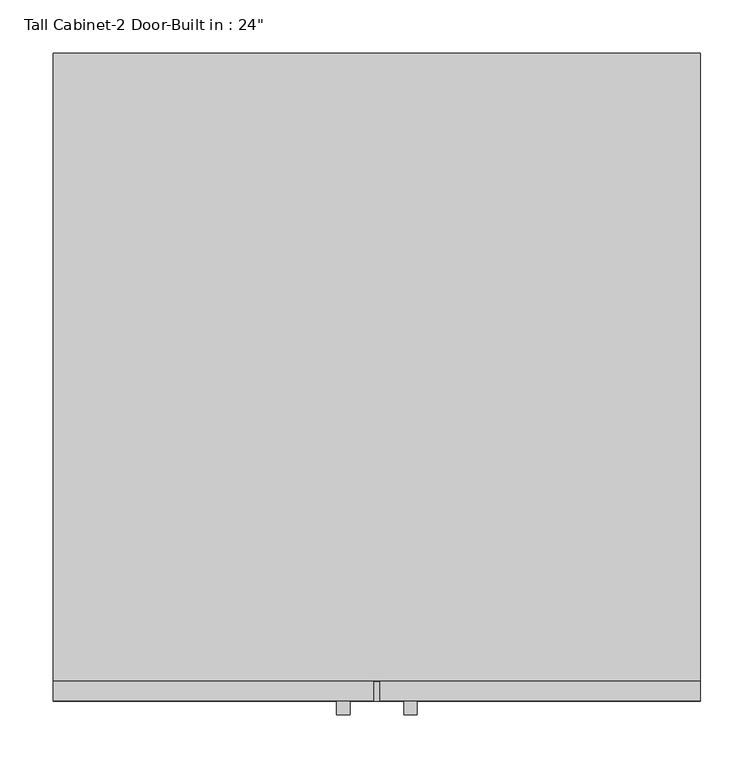
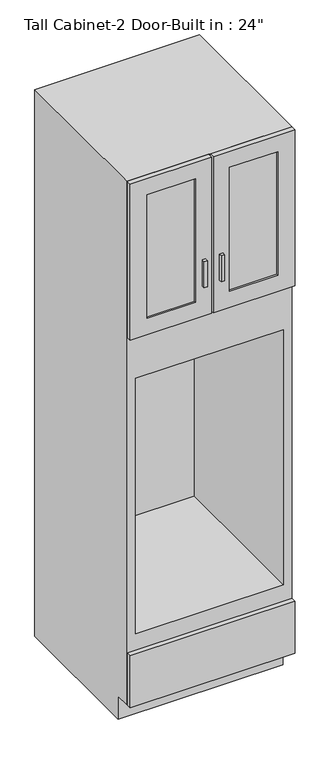
"""IFC4 building model written with IfcOpenShell, lengths in millimetres: furniture geometry."""

import ifcopenshell
import ifcopenshell.guid

model = None  # the IFC model being written
_history = None  # IfcOwnerHistory: only IFC2X3 demands one
_inside = {}  # id of a spatial element -> (the spatial element, [elements in it])
_under = {}  # id of a project, library or spatial element -> (it, [spatial elements below it])
_declared = {}  # id of a project -> (the project, [libraries it declares])
_typed = {}  # id of a type object -> (the type object, [elements of that type])
_made_of = {}  # id of a material, layer set ... -> (it, [elements and type objects made of it])


def new_model(schema):
    """Start an empty IFC model of exactly this schema.

    Asked for "IFC4X3", IfcOpenShell would pick the latest addendum, in which some entities
    have other attributes; the version numbers below select the first issue.
    IFC2X3 requires an IfcOwnerHistory on every rooted entity: one is made here for all.
    """
    global model, _history
    if schema == "IFC4X3":
        model = ifcopenshell.file(schema_version=(4, 3, 0, 0))
    else:
        model = ifcopenshell.file(schema=schema)
    _inside.clear()
    _under.clear()
    _declared.clear()
    _typed.clear()
    _made_of.clear()
    _history = None
    if model.schema == "IFC2X3":
        org = make("IfcOrganization", Name="unknown")
        user = make(
            "IfcPersonAndOrganization",
            ThePerson=make("IfcPerson", FamilyName="unknown"),
            TheOrganization=org,
        )
        app = make(
            "IfcApplication",
            ApplicationDeveloper=org,
            Version="unknown",
            ApplicationFullName="unknown",
            ApplicationIdentifier="unknown",
        )
        _history = make(
            "IfcOwnerHistory",
            OwningUser=user,
            OwningApplication=app,
            ChangeAction="ADDED",
            CreationDate=0,
        )
    return model


def make(cls, **values):
    """One entity of the class cls with the attributes given. An attribute that is None is left unset."""
    return model.create_entity(
        cls, **{name: value for name, value in values.items() if value is not None}
    )


def rooted(cls, **values):
    """An entity with a GlobalId (a new one), such as an element, a storey or a relation."""
    return make(cls, GlobalId=ifcopenshell.guid.new(), OwnerHistory=_history, **values)


def si_unit(unit_type, name, prefix=None):
    """IfcSIUnit, for example si_unit("LENGTHUNIT", "METRE", prefix="MILLI")."""
    return make("IfcSIUnit", UnitType=unit_type, Prefix=prefix, Name=name)


def assignment(units):
    """IfcUnitAssignment: the units of a project."""
    return None if units is None else make("IfcUnitAssignment", Units=units)


def point(xyz):
    """IfcCartesianPoint."""
    return None if xyz is None else make("IfcCartesianPoint", Coordinates=xyz)


def direction(xyz):
    """IfcDirection."""
    return None if xyz is None else make("IfcDirection", DirectionRatios=xyz)


def frame(location, z_axis=None, x_axis=None):
    """IfcAxis2Placement3D, a coordinate frame: its origin and axes. An axis left out is left unset."""
    return make(
        "IfcAxis2Placement3D",
        Location=point(location),
        Axis=direction(z_axis),
        RefDirection=direction(x_axis),
    )


def origin():
    """The frame at (0, 0, 0) with its axes left unset."""
    return frame((0.0, 0.0, 0.0))


def place(relative_to, where):
    """IfcLocalPlacement: puts the frame where relative to a parent placement (None: the world)."""
    return make(
        "IfcLocalPlacement", PlacementRelTo=relative_to, RelativePlacement=where
    )


def context(
    kind, dimensions, precision=None, world=None, true_north=None, identifier=None
):
    """IfcGeometricRepresentationContext, for example the 3D "Model" context."""
    return make(
        "IfcGeometricRepresentationContext",
        ContextIdentifier=identifier,
        ContextType=kind,
        CoordinateSpaceDimension=dimensions,
        Precision=precision,
        WorldCoordinateSystem=world,
        TrueNorth=true_north,
    )


def project(units=None, contexts=None):
    """IfcProject with its units and contexts."""
    return rooted(
        "IfcProject",
        Name="project",
        RepresentationContexts=contexts,
        UnitsInContext=assignment(units),
    )


def spatial(cls, under=None, at=None, **own):
    """A site, building, storey or space (cls), placed at a placement, below another one or the project."""
    s = rooted(cls, ObjectPlacement=at, **own)
    if under is not None:
        _under.setdefault(under.id(), (under, []))[1].append(s)
    return s


def polyline(points):
    """IfcPolyline through the points."""
    return make("IfcPolyline", Points=[point(p) for p in points])


def outline(outer, holes=None, kind="AREA"):
    """IfcArbitraryClosedProfileDef: a profile drawn as a closed curve; with holes, ...WithVoids."""
    if holes is None:
        return make("IfcArbitraryClosedProfileDef", ProfileType=kind, OuterCurve=outer)
    return make(
        "IfcArbitraryProfileDefWithVoids",
        ProfileType=kind,
        OuterCurve=outer,
        InnerCurves=holes,
    )


def extrude(swept, where, along, depth):
    """IfcExtrudedAreaSolid: the profile swept, set in the frame where, extruded along a direction by depth."""
    return make(
        "IfcExtrudedAreaSolid",
        SweptArea=swept,
        Position=where,
        ExtrudedDirection=direction(along),
        Depth=depth,
    )


def faces_of(points, faces, orient=None, outer=None):
    """IfcFace entities. A face is a list of loops; a loop is a list of indices into points, from 0.

    orient and outer hold one flag for each loop. By default every Orientation is true, the
    first loop of a face is its IfcFaceOuterBound and the others are IfcFaceBound.
    """
    made = []
    for i, loops in enumerate(faces):
        bounds = []
        for j, loop in enumerate(loops):
            is_outer = j == 0 if outer is None else outer[i][j]
            bounds.append(
                make(
                    "IfcFaceOuterBound" if is_outer else "IfcFaceBound",
                    Bound=make("IfcPolyLoop", Polygon=[points[k] for k in loop]),
                    Orientation=True if orient is None else orient[i][j],
                )
            )
        made.append(make("IfcFace", Bounds=bounds))
    return made


def faceted_brep(points, faces, orient=None, outer=None, voids=None):
    """IfcFacetedBrep: a solid bounded by flat faces; with voids (closed shells), ...WithVoids."""
    shared = [point(p) for p in points]
    hull = make("IfcClosedShell", CfsFaces=faces_of(shared, faces, orient, outer))
    if voids is None:
        return make("IfcFacetedBrep", Outer=hull)
    return make(
        "IfcFacetedBrepWithVoids",
        Outer=hull,
        Voids=[
            make(cls, CfsFaces=faces_of(shared, fs, o, b)) for cls, fs, o, b in voids
        ],
    )


def shape(context_of_items, identifier, shape_type, items):
    """IfcShapeRepresentation: the items that make up one representation, for example the "Body"."""
    return make(
        "IfcShapeRepresentation",
        ContextOfItems=context_of_items,
        RepresentationIdentifier=identifier,
        RepresentationType=shape_type,
        Items=items,
    )


def source(mapping_origin, context_of_items, identifier, shape_type, items):
    """IfcRepresentationMap: a shape defined once, which mapped items show again and again."""
    return make(
        "IfcRepresentationMap",
        MappingOrigin=mapping_origin,
        MappedRepresentation=shape(context_of_items, identifier, shape_type, items),
    )


def transform(
    local_origin,
    x_axis=None,
    y_axis=None,
    z_axis=None,
    scale=None,
    scale2=None,
    scale3=None,
    uniform=True,
):
    """IfcCartesianTransformationOperator3D, or its non-uniform kind. x_axis, y_axis, z_axis: its Axis1, 2, 3."""
    if uniform:
        return make(
            "IfcCartesianTransformationOperator3D",
            Axis1=direction(x_axis),
            Axis2=direction(y_axis),
            LocalOrigin=point(local_origin),
            Scale=scale,
            Axis3=direction(z_axis),
        )
    return make(
        "IfcCartesianTransformationOperator3DnonUniform",
        Axis1=direction(x_axis),
        Axis2=direction(y_axis),
        LocalOrigin=point(local_origin),
        Scale=scale,
        Axis3=direction(z_axis),
        Scale2=scale2,
        Scale3=scale3,
    )


def mapped(mapping_source, mapping_target):
    """IfcMappedItem: shows the shape of a source again, moved by a transform."""
    return make(
        "IfcMappedItem", MappingSource=mapping_source, MappingTarget=mapping_target
    )


def made_of(thing, what):
    """Note that an element or type object is made of a material, layer set ...; save() writes the relation."""
    if what is not None:
        _made_of.setdefault(what.id(), (what, []))[1].append(thing)
    return thing


def element(
    cls,
    number,
    at=None,
    inside=None,
    cuts=None,
    type_object=None,
    material=None,
    context=None,
    identifier="Body",
    shape_type=None,
    held_by="IfcProductDefinitionShape",
    body=None,
    shapes=None,
    **own,
):
    """One element of the class cls, such as IfcWall. Its Tag is "e" and its number.

    at: its placement. inside: the storey or other place that contains it. cuts: it is an
    opening in that element (IfcRelVoidsElement). A single representation is given by context,
    identifier, shape_type and body (its items); several are given by shapes. held_by: the class
    of the entity that holds the representations. save() writes the other relations.
    """
    e = rooted(cls, Tag="e%d" % number, ObjectPlacement=at, **own)
    if body is not None:
        shapes = [shape(context, identifier, shape_type, body)]
    if shapes is not None:
        e.Representation = make(held_by, Representations=shapes)
    if inside is not None:
        _inside.setdefault(inside.id(), (inside, []))[1].append(e)
    if cuts is not None:
        rooted(
            "IfcRelVoidsElement", RelatingBuildingElement=cuts, RelatedOpeningElement=e
        )
    if type_object is not None:
        _typed.setdefault(type_object.id(), (type_object, []))[1].append(e)
    return made_of(e, material)


def aggregate(whole, parts):
    """IfcRelAggregates: a whole, such as a stair, and the parts it consists of."""
    return rooted("IfcRelAggregates", RelatingObject=whole, RelatedObjects=parts)


def save(model, path):
    """Write the relations noted so far, then the file.

    IfcRelAggregates (storeys below a building ...), IfcRelContainedInSpatialStructure (elements
    in a storey), IfcRelDefinesByType, IfcRelAssociatesMaterial and IfcRelDeclares: one each for
    every whole, place, type object, material and project.
    """
    for whole, parts in _under.values():
        aggregate(whole, parts)
    for where, things in _inside.values():
        rooted(
            "IfcRelContainedInSpatialStructure",
            RelatedElements=things,
            RelatingStructure=where,
        )
    for kind, things in _typed.values():
        rooted("IfcRelDefinesByType", RelatedObjects=things, RelatingType=kind)
    for what, things in _made_of.values():
        rooted("IfcRelAssociatesMaterial", RelatedObjects=things, RelatingMaterial=what)
    for by, libraries in _declared.values():
        rooted("IfcRelDeclares", RelatingContext=by, RelatedDefinitions=libraries)
    model.write(path)


def furniture_1eba2136(model_context):
    return source(origin(), model_context, "Body", "SolidModel", [
        faceted_brep([(323.5377049, -590.55, 90.4875), (323.5377049, -590.55, 2135.1875), (-286.0622951, -590.55, 2135.1875), (-286.0622951, -590.55, 90.4875), (-267.0122951, -590.55, 2116.1375), (304.4877049, -590.55, 2116.1375), (304.4877049, -590.55, 1525.5875), (-267.0122951, -590.55, 1525.5875), (291.7877049, -590.55, 357.1875), (-254.3122951, -590.55, 357.1875), (-254.3122951, -590.55, 1354.1375), (291.7877049, -590.55, 1354.1375), (-286.0622951, 0.0, 2135.1875), (323.5377049, 0.0, 2135.1875), (323.5377049, 0.0, 0.0), (-286.0622951, 0.0, 0.0), (323.5377049, -533.4, 90.4875), (323.5377049, -533.4, 0.0), (-286.0622951, -533.4, 0.0), (-286.0622951, -533.4, 90.4875), (304.4877049, -19.05, 2116.1375), (304.4877049, -19.05, 1525.5875), (-267.0122951, -19.05, 1525.5875), (-267.0122951, -19.05, 2116.1375), (291.7877049, -19.05, 357.1875), (-254.3122951, -19.05, 357.1875), (-254.3122951, -19.05, 1354.1375), (291.7877049, -19.05, 1354.1375)], [[[0, 1, 2, 3], [4, 5, 6, 7], [8, 9, 10, 11]], [[12, 13, 14, 15]], [[1, 0, 16, 17, 14, 13]], [[2, 1, 13, 12]], [[3, 2, 12, 15, 18, 19]], [[0, 3, 19, 16]], [[6, 5, 20, 21]], [[4, 7, 22, 23]], [[5, 4, 23, 20]], [[14, 17, 18, 15]], [[18, 17, 16, 19]], [[7, 6, 21, 22]], [[9, 8, 24, 25]], [[10, 9, 25, 26]], [[11, 10, 26, 27]], [[8, 11, 27, 24]], [[21, 20, 23, 22]], [[25, 24, 27, 26]]]),
        extrude(outline(polyline([(323.5377049, -609.6), (-286.0622951, -609.6), (-286.0622951, -590.55), (323.5377049, -590.55), (323.5377049, -609.6)])), frame((0.0, 0.0, 90.4875), z_axis=(0.0, 0.0, 1.0), x_axis=(1.0, 0.0, 0.0)), (0.0, 0.0, 1.0), 203.2),
        extrude(outline(polyline([(2135.1875, 15.5627049), (2135.1875, -286.0622951), (1525.5875, -286.0622951), (1525.5875, 15.5627049), (2135.1875, 15.5627049)]), holes=[polyline([(2071.6875, -44.7622951), (1589.0875, -44.7622951), (1589.0875, -222.5622951), (2071.6875, -222.5622951), (2071.6875, -44.7622951)])]), frame((0.0, -609.6, 0.0), z_axis=(0.0, 1.0, 0.0), x_axis=(0.0, 0.0, 1.0)), (0.0, 0.0, 1.0), 19.05),
        extrude(outline(polyline([(2135.1875, 21.9127049), (1525.5875, 21.9127049), (1525.5875, 323.5377049), (2135.1875, 323.5377049), (2135.1875, 21.9127049)]), holes=[polyline([(2071.6875, 260.0377049), (1589.0875, 260.0377049), (1589.0875, 82.2377049), (2071.6875, 82.2377049), (2071.6875, 260.0377049)])]), frame((0.0, -609.6, 0.0), z_axis=(0.0, 1.0, 0.0), x_axis=(0.0, 0.0, 1.0)), (0.0, 0.0, 1.0), 19.05),
        extrude(outline(polyline([(323.5377049, -609.6), (-286.0622951, -609.6), (-286.0622951, -590.55), (323.5377049, -590.55), (323.5377049, -609.6)])), frame((0.0, 0.0, 90.4875), z_axis=(0.0, 0.0, 1.0), x_axis=(1.0, 0.0, 0.0)), (0.0, 0.0, 1.0), 203.2),
        extrude(outline(polyline([(-6.6622951, -622.3), (-19.1945267, -622.3), (-19.1945267, -609.6), (-6.6622951, -609.6), (-6.6622951, -622.3)])), frame((0.0, 0.0, 1645.6417867), z_axis=(0.0, 0.0, 1.0), x_axis=(1.0, 0.0, 0.0)), (0.0, 0.0, 1.0), 101.6),
        extrude(outline(polyline([(56.6699365, -622.3), (44.1377049, -622.3), (44.1377049, -609.6), (56.6699365, -609.6), (56.6699365, -622.3)])), frame((0.0, 0.0, 1645.6417867), z_axis=(0.0, 0.0, 1.0), x_axis=(1.0, 0.0, 0.0)), (0.0, 0.0, 1.0), 101.6),
        extrude(outline(polyline([(-44.7622951, -603.25), (-222.5622951, -603.25), (-222.5622951, -596.9), (-44.7622951, -596.9), (-44.7622951, -603.25)])), frame((0.0, 0.0, 1589.0875), z_axis=(0.0, 0.0, 1.0), x_axis=(1.0, 0.0, 0.0)), (0.0, 0.0, 1.0), 482.6),
        extrude(outline(polyline([(260.0377049, -603.25), (82.2377049, -603.25), (82.2377049, -596.9), (260.0377049, -596.9), (260.0377049, -603.25)])), frame((0.0, 0.0, 1589.0875), z_axis=(0.0, 0.0, 1.0), x_axis=(1.0, 0.0, 0.0)), (0.0, 0.0, 1.0), 482.6),
    ])


if __name__ == "__main__":
    model = new_model("IFC4")
    model_context = context("Model", 3, world=origin())
    ifc_project = project(units=[si_unit("LENGTHUNIT", "METRE", prefix="MILLI")], contexts=[model_context])
    site = spatial("IfcSite", under=ifc_project)
    building = spatial("IfcBuilding", under=site)
    placement = place(None, origin())
    furniture_shape = furniture_1eba2136(model_context)
    element("IfcFurniture", 1, ObjectType="Tall Cabinet-2 Door-Built in : 24\"", at=placement, inside=building, context=model_context, shape_type="MappedRepresentation", body=[
        mapped(furniture_shape, transform((0.0, 0.0, 0.0), x_axis=(1.0, 0.0, 0.0), y_axis=(0.0, 1.0, 0.0), z_axis=(0.0, 0.0, 1.0))),
    ])
    save(model, "model.ifc")

# Revit data of these elements
# Type "Tall Cabinet-2 Door-Built in : 24\""
#   Assembly Code = "C1030410"
#   Type Comments = "21.5\"w 39.75\"h built-in"
#   Height = 7' - 0"
#   Depth = 2' - 0"
#   Height-Base of Built-in = 1' - 2"
#   Height-Built-in = 3' - 3 1/4"
#   Height-Upper Cabinet = 2' - 0"
#   Toe Depth = 0' - 3"
#   Toe Height = 0' - 3 1/2"
#   Width = 2' - 0"
#   Cabinet Material = none
#   Door/Drawer Material = none
#   Handle Material = Cabinets - Handles
#   Panel Material = Glass
# Element 1 (IfcFurniture, "Tall Cabinet-2 Door-Built in : 24\"")
#   Materials on its faces: "Cabinets", "Cabinets - Handles", "Glass"
# Materials
#   "Cabinets - Handles": class "Metal", colour RGB 57 57 57, transparency 0
#   "Glass": class "Glass", colour RGB 0 128 192, transparency 0.75, Description = "Soda Lime Glass", Cost = 0
#   "Cabinets": class "Miscellaneous", colour RGB 249 249 249, transparency 0
